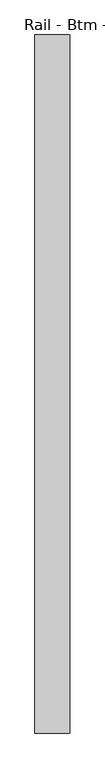
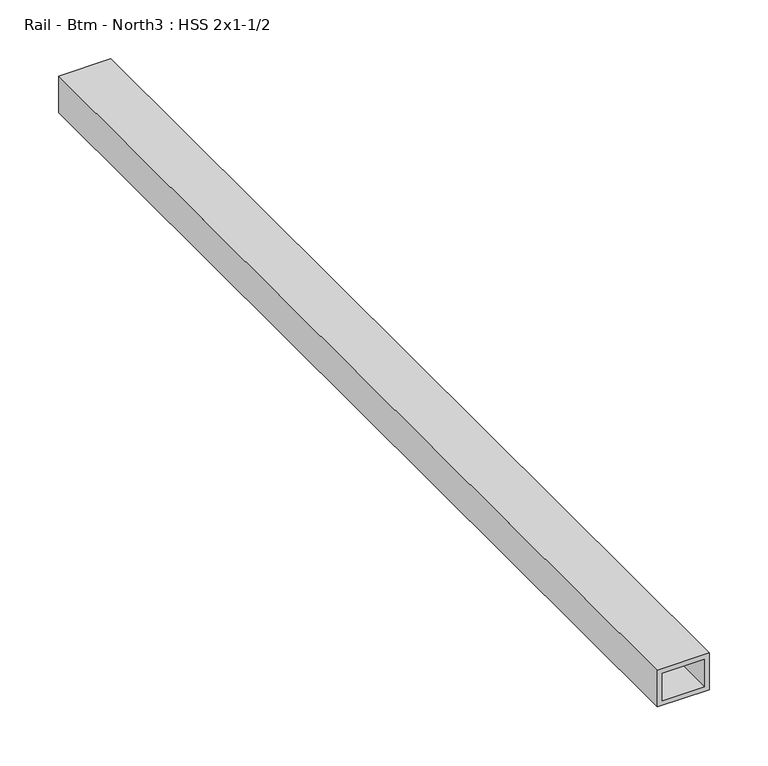
"""IFC4 building model written with IfcOpenShell, lengths in millimetres: proxy geometry, Rail - Btm - North3 : HSS 2x1-1/2."""

from ifc_helpers import new_model, si_unit, frame, origin, place, context, project, spatial, polyline, outline, extrude, source, transform, mapped, element, save


def rail_btm_north3_hss_2x1_1_2_782f6166(model_context):
    return source(origin(), model_context, "Body", "SweptSolid", [
        extrude(outline(polyline([(50.8, 587416.6934739), (88.9, 587416.6934739), (88.9, 587365.8934739), (50.8, 587365.8934739), (50.8, 587416.6934739)]), holes=[polyline([(84.1375, 587411.9309739), (55.5625, 587411.9309739), (55.5625, 587370.6559739), (84.1375, 587370.6559739), (84.1375, 587411.9309739)])]), frame((0.0, -535163.4663841, 0.0), z_axis=(0.0, 1.0, 0.0), x_axis=(0.0, 0.0, 1.0)), (0.0, 0.0, 1.0), 1016.0),
    ])


if __name__ == "__main__":
    model = new_model("IFC4")
    model_context = context("Model", 3, world=origin())
    ifc_project = project(units=[si_unit("LENGTHUNIT", "METRE", prefix="MILLI")], contexts=[model_context])
    site = spatial("IfcSite", under=ifc_project)
    building = spatial("IfcBuilding", under=site)
    placement = place(None, origin())
    rail_btm_north3_hss_2x1_1_2_shape = rail_btm_north3_hss_2x1_1_2_782f6166(model_context)
    element("IfcBuildingElementProxy", 1, Name="Rail - Btm - North3 : HSS 2x1-1/2", ObjectType="Rail - Btm - North3 : HSS 2x1-1/2", at=placement, inside=building, context=model_context, shape_type="MappedRepresentation", body=[
        mapped(rail_btm_north3_hss_2x1_1_2_shape, transform((0.0, 0.0, 0.0), x_axis=(1.0, 0.0, 0.0), y_axis=(0.0, 1.0, 0.0), z_axis=(0.0, 0.0, 1.0))),
    ])
    save(model, "model.ifc")

# Revit data of these elements
# Element 1 (IfcBuildingElementProxy, "Rail - Btm - North3 : HSS 2x1-1/2")
#   Materials on its faces: "1-1/2\"X2\" GALV. STL HSS TUBING"
# Materials
#   "1-1/2\"X2\" GALV. STL HSS TUBING": class "Generic", colour RGB 211 211 207, transparency 0, Cost = 0
